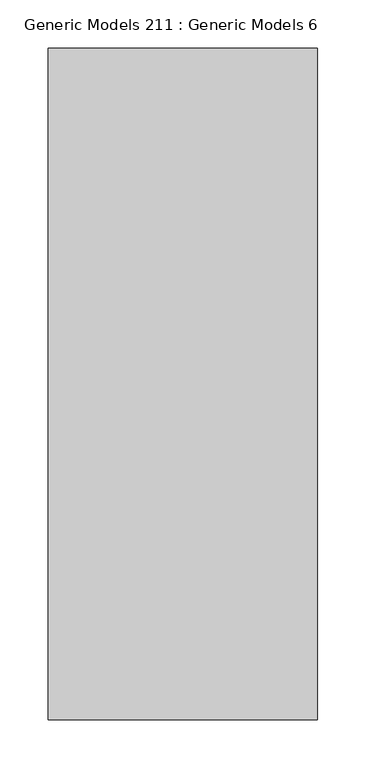
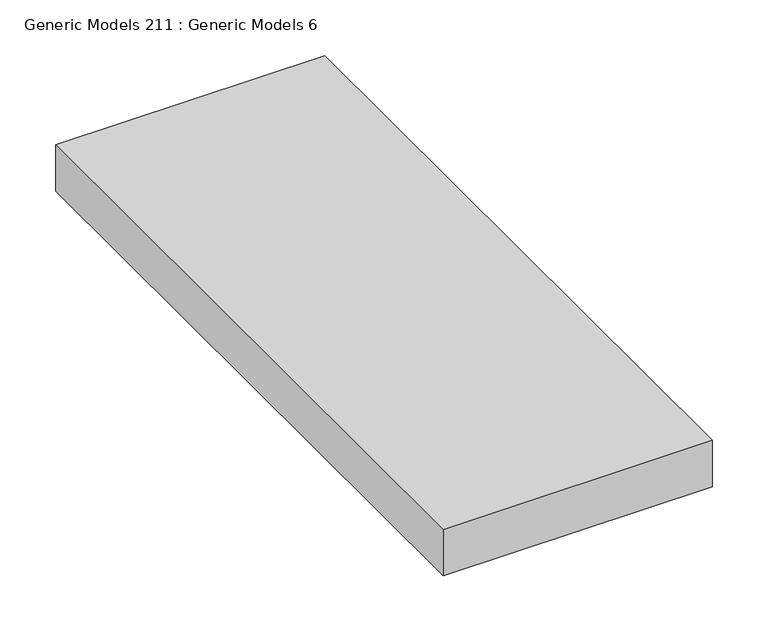
"""IFC4 building model written with IfcOpenShell, lengths in millimetres: proxy geometry, Generic Models 211 : Generic Models 6."""

from ifc_helpers import new_model, si_unit, frame, origin, place, context, project, spatial, polyline, outline, extrude, source, transform, mapped, element, save


def generic_models_211_generic_models_6_2777844f(model_context):
    return source(origin(), model_context, "Body", "SweptSolid", [
        extrude(outline(polyline([(190.3263704, 1095.7884092), (469.7263704, 1095.7884092), (469.7263704, 399.7309662), (190.3263704, 399.7309662), (190.3263704, 1095.7884092)])), frame((0.0, 0.0, 126599.696), z_axis=(0.0, 0.0, 1.0), x_axis=(1.0, 0.0, 0.0)), (0.0, 0.0, 1.0), 50.8),
    ])


if __name__ == "__main__":
    model = new_model("IFC4")
    model_context = context("Model", 3, world=origin())
    ifc_project = project(units=[si_unit("LENGTHUNIT", "METRE", prefix="MILLI")], contexts=[model_context])
    site = spatial("IfcSite", under=ifc_project)
    building = spatial("IfcBuilding", under=site)
    placement = place(None, origin())
    generic_models_211_generic_models_6_shape = generic_models_211_generic_models_6_2777844f(model_context)
    element("IfcBuildingElementProxy", 1, Name="Generic Models 211 : Generic Models 6", ObjectType="Generic Models 211 : Generic Models 6", at=placement, inside=building, context=model_context, shape_type="MappedRepresentation", body=[
        mapped(generic_models_211_generic_models_6_shape, transform((0.0, 0.0, 0.0), x_axis=(1.0, 0.0, 0.0), y_axis=(0.0, 1.0, 0.0), z_axis=(0.0, 0.0, 1.0))),
    ])
    save(model, "model.ifc")

# Revit data of these elements
# Element 1 (IfcBuildingElementProxy, "Generic Models 211 : Generic Models 6")
#   Materials on its faces: "_HARDWOOD TREADS, SPECIES AND FINISH PER OWNER"
# Materials
#   "_HARDWOOD TREADS, SPECIES AND FINISH PER OWNER": class "Generic", colour RGB 177 130 114, transparency 0, Cost = 0
